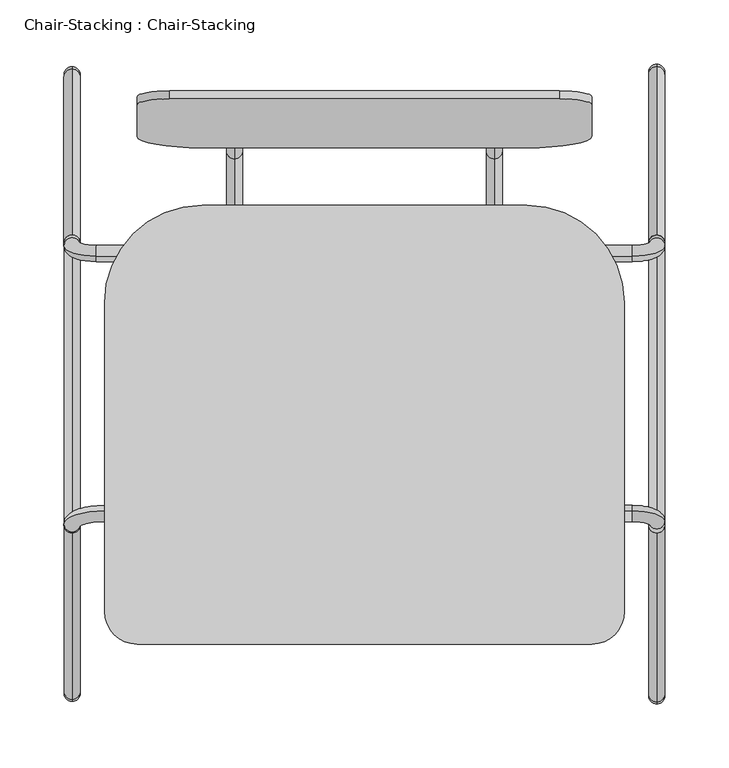
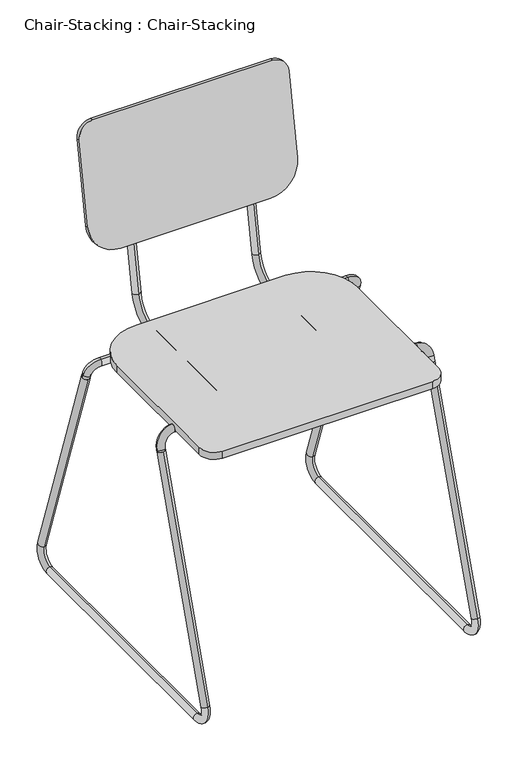
"""IFC4 building model written with IfcOpenShell, lengths in millimetres: furniture geometry, Chair-Stacking : Chair-Stacking."""

from ifc_helpers import new_model, si_unit, point, frame, frame_2d, origin, place, context, project, spatial, polyline, circle_curve, ellipse_curve, trimmed, segment, composite_curve, outline, extrude, source, transform, mapped, element, save
from ifc_brep_helpers import plane_surface, cylinder_surface, revolved_surface, advanced_brep


def chair_stacking_chair_stacking_89a83372(model_context):
    return source(origin(), model_context, "Body", "SolidModel", [
        advanced_brep(
        [(-280.6491803, -213.2656675, 431.8), (-280.6491803, -213.2656675, 444.5), (-280.6491803, 23.0277124, 444.5), (-280.6491803, 23.0277124, 431.8), (-280.6491803, 66.802417, 481.2313385), (-280.6491803, 79.3094755, 479.0260066), (-280.6491803, 119.2282049, 705.4163709), (-280.6491803, 106.7211464, 707.6217027)],
        [
            (0, 1, circle_curve(frame((-280.6491803, -213.2656675, 438.15), z_axis=(0.0, -1.0, 0.0), x_axis=(0.0, 0.0, 1.0)), 6.35)),
            (1, 0, circle_curve(frame((-280.6491803, -213.2656675, 438.15), z_axis=(0.0, -1.0, 0.0), x_axis=(0.0, 0.0, 1.0)), 6.35)),
            (1, 2),
            (2, 3, circle_curve(frame((-280.6491803, 23.0277124, 438.15), z_axis=(0.0, -1.0, 0.0), x_axis=(0.0, 0.0, 1.0)), 6.35)),
            (3, 0),
            (3, 2, circle_curve(frame((-280.6491803, 23.0277124, 438.15), z_axis=(0.0, -1.0, 0.0), x_axis=(0.0, 0.0, 1.0)), 6.35)),
            (4, 5, circle_curve(frame((-280.6491803, 73.0559463, 480.1286726), z_axis=(0.0, -0.17364817766693444, -0.9848077530122074), x_axis=(0.0, -0.9848077530122074, 0.17364817766693444)), 6.35)),
            (5, 3, circle_curve(frame((-280.6491803, 23.0277124, 488.95), z_axis=(-1.0, 0.0, 0.0), x_axis=(0.0, 0.0, -1.0)), 57.15)),
            (2, 4, circle_curve(frame((-280.6491803, 23.0277124, 488.95), z_axis=(1.0, 0.0, 0.0), x_axis=(0.0, 0.0, -1.0)), 44.45)),
            (5, 4, circle_curve(frame((-280.6491803, 73.0559463, 480.1286726), z_axis=(0.0, -0.17364817766693444, -0.9848077530122074), x_axis=(0.0, -0.9848077530122074, 0.17364817766693444)), 6.35)),
            (6, 7, circle_curve(frame((-280.6491803, 112.9746757, 706.5190368), z_axis=(0.0, 0.1736481776669348, 0.9848077530122074), x_axis=(0.0, -0.9848077530122074, 0.1736481776669348)), 6.35)),
            (7, 6, circle_curve(frame((-280.6491803, 112.9746757, 706.5190368), z_axis=(0.0, 0.1736481776669348, 0.9848077530122074), x_axis=(0.0, -0.9848077530122074, 0.1736481776669348)), 6.35)),
            (4, 7),
            (6, 5),
        ],
        [
            plane_surface(frame((-286.9991803, -213.2656675, 438.15), z_axis=(0.0, -1.0, 0.0), x_axis=(0.0, 0.0, -1.0))),
            cylinder_surface(frame((-280.6491803, -213.2656675, 438.15), z_axis=(0.0, -1.0, 0.0), x_axis=(0.0, 0.0, 1.0)), 6.35),
            revolved_surface(trimmed(ellipse_curve(frame((-280.6491803, 23.0277124, 438.15), z_axis=(0.0, 1.0, 0.0), x_axis=(0.0, 0.0, 1.0)), 6.35, 6.35), [point((-280.6491803, 23.0277124, 431.8))], [point((-280.6491803, 23.0277124, 444.5))], True, "CARTESIAN"), (-280.6491803, 23.0277124, 488.95), (-1.0, 0.0, 0.0)),
            revolved_surface(trimmed(ellipse_curve(frame((-280.6491803, 23.0277124, 438.15), z_axis=(0.0, 1.0, 0.0), x_axis=(0.0, 0.0, 1.0)), 6.35, 6.35), [point((-280.6491803, 23.0277124, 444.5))], [point((-280.6491803, 23.0277124, 431.8))], True, "CARTESIAN"), (-280.6491803, 23.0277124, 488.95), (-1.0, 0.0, 0.0)),
            plane_surface(frame((-280.6491803, 119.2282049, 705.4163709), z_axis=(0.0, 0.17364817766692842, 0.9848077530122085), x_axis=(1.0, 0.0, 0.0))),
            cylinder_surface(frame((-280.6491803, 73.0559463, 480.1286726), z_axis=(0.0, -0.1736481776669348, -0.9848077530122074), x_axis=(0.0, -0.9848077530122074, 0.1736481776669348)), 6.35),
        ],
        [
            (0, [[1, 2]]),
            (1, [[3, 4, 5, -2]]),
            (1, [[-5, 6, -3, -1]]),
            (2, [[7, 8, -4, 9]]),
            (3, [[10, -9, -6, -8]]),
            (4, [[11, 12]]),
            (5, [[13, -11, 14, -7]]),
            (5, [[-14, -12, -13, -10]]),
        ],
    ),
        advanced_brep(
        [(-77.4491803, -213.2656675, 431.8), (-77.4491803, -213.2656675, 444.5), (-77.4491803, 23.0277124, 444.5), (-77.4491803, 23.0277124, 431.8), (-77.4491803, 66.802417, 481.2313385), (-77.4491803, 79.3094755, 479.0260066), (-77.4491803, 118.9339087, 703.7473341), (-77.4491803, 106.4268502, 705.9526659)],
        [
            (0, 1, circle_curve(frame((-77.4491803, -213.2656675, 438.15), z_axis=(0.0, -1.0, 0.0), x_axis=(0.0, 0.0, 1.0)), 6.35)),
            (1, 0, circle_curve(frame((-77.4491803, -213.2656675, 438.15), z_axis=(0.0, -1.0, 0.0), x_axis=(0.0, 0.0, 1.0)), 6.35)),
            (1, 2),
            (2, 3, circle_curve(frame((-77.4491803, 23.0277124, 438.15), z_axis=(0.0, -1.0, 0.0), x_axis=(0.0, 0.0, 1.0)), 6.35)),
            (3, 0),
            (3, 2, circle_curve(frame((-77.4491803, 23.0277124, 438.15), z_axis=(0.0, -1.0, 0.0), x_axis=(0.0, 0.0, 1.0)), 6.35)),
            (4, 5, circle_curve(frame((-77.4491803, 73.0559463, 480.1286726), z_axis=(0.0, -0.1736481776669372, -0.9848077530122068), x_axis=(0.0, -0.9848077530122068, 0.1736481776669372)), 6.35)),
            (5, 3, circle_curve(frame((-77.4491803, 23.0277124, 488.95), z_axis=(-1.0, 0.0, 0.0), x_axis=(0.0, 0.0, -1.0)), 57.15)),
            (2, 4, circle_curve(frame((-77.4491803, 23.0277124, 488.95), z_axis=(1.0, 0.0, 0.0), x_axis=(0.0, 0.0, -1.0)), 44.45)),
            (5, 4, circle_curve(frame((-77.4491803, 73.0559463, 480.1286726), z_axis=(0.0, -0.1736481776669385, -0.9848077530122066), x_axis=(0.0, -0.9848077530122066, 0.1736481776669385)), 6.35)),
            (6, 7, circle_curve(frame((-77.4491803, 112.6803794, 704.85), z_axis=(0.0, 0.17364817766693896, 0.9848077530122066), x_axis=(0.0, -0.9848077530122066, 0.17364817766693896)), 6.35)),
            (7, 6, circle_curve(frame((-77.4491803, 112.6803794, 704.85), z_axis=(0.0, 0.17364817766693896, 0.9848077530122066), x_axis=(0.0, -0.9848077530122066, 0.17364817766693896)), 6.35)),
            (4, 7),
            (6, 5),
        ],
        [
            plane_surface(frame((-83.7991803, -213.2656675, 438.15), z_axis=(0.0, -1.0, 0.0), x_axis=(0.0, 0.0, -1.0))),
            cylinder_surface(frame((-77.4491803, -213.2656675, 438.15), z_axis=(0.0, -1.0, 0.0), x_axis=(0.0, 0.0, 1.0)), 6.35),
            revolved_surface(trimmed(ellipse_curve(frame((-77.4491803, 23.0277124, 438.15), z_axis=(0.0, 1.0, 0.0), x_axis=(0.0, 0.0, 1.0)), 6.35, 6.35), [point((-77.4491803, 23.0277124, 431.8))], [point((-77.4491803, 23.0277124, 444.5))], True, "CARTESIAN"), (-77.4491803, 23.0277124, 488.95), (-1.0, 0.0, 0.0)),
            revolved_surface(trimmed(ellipse_curve(frame((-77.4491803, 23.0277124, 438.15), z_axis=(0.0, 1.0, 0.0), x_axis=(0.0, 0.0, 1.0)), 6.35, 6.35), [point((-77.4491803, 23.0277124, 444.5))], [point((-77.4491803, 23.0277124, 431.8))], True, "CARTESIAN"), (-77.4491803, 23.0277124, 488.95), (-1.0, 0.0, 0.0)),
            plane_surface(frame((-77.4491803, 118.9339087, 703.7473341), z_axis=(0.0, 0.17364817766692892, 0.9848077530122084), x_axis=(1.0, 0.0, 0.0))),
            cylinder_surface(frame((-77.4491803, 73.0559463, 480.1286726), z_axis=(0.0, -0.17364817766693896, -0.9848077530122066), x_axis=(0.0, -0.9848077530122066, 0.17364817766693896)), 6.35),
        ],
        [
            (0, [[1, 2]]),
            (1, [[3, 4, 5, -2]]),
            (1, [[-5, 6, -3, -1]]),
            (2, [[7, 8, -4, 9]]),
            (3, [[10, -9, -6, -8]]),
            (4, [[11, 12]]),
            (5, [[13, -11, 14, -7]]),
            (5, [[-14, -12, -13, -10]]),
        ],
    ),
        extrude(outline(composite_curve([segment(polyline([(-1.2491803, -312.1314636), (-356.8491803, -312.1314636)]), True, "CONTINUOUS"), segment(trimmed(circle_curve(frame_2d((-356.8491803, -286.7314636)), 25.4), [point((-356.8491803, -312.1314636))], [point((-382.2491803, -286.7314636))], False, "CARTESIAN"), True, "CONTINUOUS"), segment(polyline([(-382.2491803, -286.7314636), (-382.2491803, -45.4314636)]), True, "CONTINUOUS"), segment(trimmed(circle_curve(frame_2d((-306.0491803, -45.4314636)), 76.2), [point((-382.2491803, -45.4314636))], [point((-306.0491803, 30.7685364))], False, "CARTESIAN"), True, "CONTINUOUS"), segment(polyline([(-306.0491803, 30.7685364), (-52.0491803, 30.7685364)]), True, "CONTINUOUS"), segment(trimmed(circle_curve(frame_2d((-52.0491803, -45.4314636)), 76.2), [point((-52.0491803, 30.7685364))], [point((24.1508197, -45.4314636))], False, "CARTESIAN"), True, "CONTINUOUS"), segment(polyline([(24.1508197, -45.4314636), (24.1508197, -286.7314636)]), True, "CONTINUOUS"), segment(trimmed(circle_curve(frame_2d((-1.2491803, -286.7314636)), 25.4), [point((24.1508197, -286.7314636))], [point((-1.2491803, -312.1314636))], False, "CARTESIAN"), True, "CONTINUOUS")], self_intersect=False)), frame((0.0, 0.0, 444.5), z_axis=(0.0, 0.0, 1.0), x_axis=(1.0, 0.0, 0.0)), (0.0, 0.0, 1.0), 12.7),
        extrude(outline(composite_curve([segment(trimmed(circle_curve(frame_2d((-304.8, 25.4)), 25.4), [point((-304.8, 0.0))], [point((-330.2, 25.4))], False, "CARTESIAN"), True, "CONTINUOUS"), segment(polyline([(-330.2, 25.4), (-330.2, 168.3013626)]), True, "CONTINUOUS"), segment(trimmed(circle_curve(frame_2d((-279.4, 168.3013626)), 50.8), [point((-330.2, 168.3013626))], [point((-279.4, 219.1013626))], False, "CARTESIAN"), True, "CONTINUOUS"), segment(polyline([(-279.4, 219.1013626), (-25.4, 219.1013626)]), True, "CONTINUOUS"), segment(trimmed(circle_curve(frame_2d((-25.4, 168.3013626)), 50.8), [point((-25.4, 219.1013626))], [point((25.4, 168.3013626))], False, "CARTESIAN"), True, "CONTINUOUS"), segment(polyline([(25.4, 168.3013626), (25.4, 25.4)]), True, "CONTINUOUS"), segment(trimmed(circle_curve(frame_2d((0.0, 25.4)), 25.4), [point((25.4, 25.4))], [point((0.0, 0.0))], False, "CARTESIAN"), True, "CONTINUOUS"), segment(polyline([(0.0, 0.0), (-304.8, 0.0)]), True, "CONTINUOUS")], self_intersect=False)), frame((-331.4491803, 119.9531376, 782.6640535), z_axis=(0.0, -0.9848077530122084, 0.17364817766692858), x_axis=(-1.0, 0.0, 0.0)), (0.0, 0.0, 1.0), 6.35),
        advanced_brep(
        [(55.9008197, -219.2327758, 419.1211728), (43.2008197, -219.2327758, 419.1211728), (43.2008197, -216.3017292, 427.6700586), (55.9008197, -216.3017292, 427.6700586), (30.5008197, -212.1828103, 439.6835721), (30.5008197, -208.0638914, 451.6970857), (-382.2491803, -212.1828103, 439.6835721), (-382.2491803, -208.0638914, 451.6970857), (-401.2991803, -218.3611887, 421.6633019), (-413.9991803, -218.3611887, 421.6633019), (-413.9991803, -219.2424531, 419.0929473), (-401.2991803, -219.2424531, 419.0929473)],
        [
            (0, 1, circle_curve(frame((49.5508197, -219.2327758, 419.1211728), z_axis=(0.0, -0.32432432432432967, -0.9459459459459442), x_axis=(-1.0, 0.0, 0.0)), 6.35)),
            (1, 0, circle_curve(frame((49.5508197, -219.2327758, 419.1211728), z_axis=(0.0, -0.32432432432432967, -0.9459459459459442), x_axis=(-1.0, 0.0, 0.0)), 6.35)),
            (1, 2),
            (2, 3, circle_curve(frame((49.5508197, -216.3017292, 427.6700586), z_axis=(0.0, -0.32432432432432967, -0.9459459459459442), x_axis=(-1.0, 0.0, 0.0)), 6.35)),
            (3, 0),
            (3, 2, circle_curve(frame((49.5508197, -216.3017292, 427.6700586), z_axis=(0.0, -0.32432432432432967, -0.9459459459459442), x_axis=(-1.0, 0.0, 0.0)), 6.35)),
            (4, 5, circle_curve(frame((30.5008197, -210.1233509, 445.6903289), z_axis=(1.0, 0.0, 0.0), x_axis=(0.0, -0.32432432432432745, -0.9459459459459449)), 6.35)),
            (5, 3, circle_curve(frame((30.5008197, -216.3017292, 427.6700586), z_axis=(0.0, 0.9459459459459447, -0.3243243243243281), x_axis=(1.0, 0.0, 0.0)), 25.4)),
            (2, 4, circle_curve(frame((30.5008197, -216.3017292, 427.6700586), z_axis=(0.0, -0.9459459459459447, 0.3243243243243281), x_axis=(1.0, 0.0, 0.0)), 12.7)),
            (5, 4, circle_curve(frame((30.5008197, -210.1233509, 445.6903289), z_axis=(1.0, 0.0, 0.0), x_axis=(0.0, -0.32432432432432745, -0.9459459459459449)), 6.35)),
            (4, 6),
            (6, 7, circle_curve(frame((-382.2491803, -210.1233509, 445.6903289), z_axis=(1.0, 0.0, 0.0), x_axis=(0.0, -0.32432432432432745, -0.9459459459459449)), 6.35)),
            (7, 5),
            (7, 6, circle_curve(frame((-382.2491803, -210.1233509, 445.6903289), z_axis=(1.0, 0.0, 0.0), x_axis=(0.0, -0.32432432432432745, -0.9459459459459449)), 6.35)),
            (8, 9, circle_curve(frame((-407.6491803, -218.3611887, 421.6633019), z_axis=(0.0, 0.324324324324328, 0.9459459459459447), x_axis=(1.0000000000000002, 0.0, 0.0)), 6.35)),
            (9, 7, circle_curve(frame((-382.2491803, -218.3611887, 421.6633019), z_axis=(0.0, 0.9459459459459447, -0.3243243243243281), x_axis=(0.0, 0.3243243243243281, 0.9459459459459447)), 31.75)),
            (6, 8, circle_curve(frame((-382.2491803, -218.3611887, 421.6633019), z_axis=(0.0, -0.9459459459459447, 0.3243243243243281), x_axis=(0.0, 0.3243243243243281, 0.9459459459459447)), 19.05)),
            (9, 8, circle_curve(frame((-407.6491803, -218.3611887, 421.6633019), z_axis=(0.0, 0.324324324324328, 0.9459459459459447), x_axis=(1.0000000000000002, 0.0, 0.0)), 6.35)),
            (10, 11, circle_curve(frame((-407.6491803, -219.2424531, 419.0929473), z_axis=(0.0, -0.32432432432432784, -0.9459459459459449), x_axis=(1.0, 0.0, 0.0)), 6.35)),
            (11, 10, circle_curve(frame((-407.6491803, -219.2424531, 419.0929473), z_axis=(0.0, -0.32432432432432784, -0.9459459459459449), x_axis=(1.0, 0.0, 0.0)), 6.35)),
            (8, 11),
            (10, 9),
        ],
        [
            plane_surface(frame((49.5508197, -213.226019, 417.0617133), z_axis=(0.0, -0.32432432432433117, -0.9459459459459437), x_axis=(1.0, 0.0, 0.0))),
            cylinder_surface(frame((49.5508197, -219.2327758, 419.1211728), z_axis=(0.0, -0.32432432432432967, -0.9459459459459442), x_axis=(-1.0, 0.0, 0.0)), 6.35),
            revolved_surface(trimmed(ellipse_curve(frame((49.5508197, -216.3017292, 427.6700586), z_axis=(0.0, 0.32432432432432823, 0.9459459459459447), x_axis=(-1.0, 0.0, 0.0)), 6.35, 6.35), [point((55.9008197, -216.3017292, 427.6700586))], [point((43.2008197, -216.3017292, 427.6700586))], True, "CARTESIAN"), (30.5008197, -216.3017292, 427.6700586), (0.0, 0.9459459459459447, -0.3243243243243281)),
            revolved_surface(trimmed(ellipse_curve(frame((49.5508197, -216.3017292, 427.6700586), z_axis=(0.0, 0.32432432432432823, 0.9459459459459447), x_axis=(-1.0, 0.0, 0.0)), 6.35, 6.35), [point((43.2008197, -216.3017292, 427.6700586))], [point((55.9008197, -216.3017292, 427.6700586))], True, "CARTESIAN"), (30.5008197, -216.3017292, 427.6700586), (0.0, 0.9459459459459447, -0.3243243243243281)),
            cylinder_surface(frame((30.5008197, -210.1233509, 445.6903289), z_axis=(1.0, 0.0, 0.0), x_axis=(0.0, -0.32432432432432745, -0.9459459459459449)), 6.35),
            revolved_surface(trimmed(ellipse_curve(frame((-382.2491803, -210.1233509, 445.6903289), z_axis=(-1.0000000000000002, 0.0, 0.0), x_axis=(0.0, -0.3243243243243276, -0.9459459459459449)), 6.35, 6.35), [point((-382.2491803, -208.0638914, 451.6970857))], [point((-382.2491803, -212.1828103, 439.6835721))], True, "CARTESIAN"), (-382.2491803, -218.3611887, 421.6633019), (0.0, 0.9459459459459447, -0.3243243243243281)),
            revolved_surface(trimmed(ellipse_curve(frame((-382.2491803, -210.1233509, 445.6903289), z_axis=(-1.0000000000000002, 0.0, 0.0), x_axis=(0.0, -0.3243243243243276, -0.9459459459459449)), 6.35, 6.35), [point((-382.2491803, -212.1828103, 439.6835721))], [point((-382.2491803, -208.0638914, 451.6970857))], True, "CARTESIAN"), (-382.2491803, -218.3611887, 421.6633019), (0.0, 0.9459459459459447, -0.3243243243243281)),
            plane_surface(frame((-407.6491803, -225.2492099, 421.1524068), z_axis=(0.0, -0.3243243243243264, -0.9459459459459453), x_axis=(1.0, 0.0, 0.0))),
            cylinder_surface(frame((-407.6491803, -218.3611887, 421.6633019), z_axis=(0.0, 0.3243243243243278, 0.9459459459459447), x_axis=(1.0, 0.0, 0.0)), 6.35),
        ],
        [
            (0, [[1, 2]]),
            (1, [[3, 4, 5, -2]]),
            (1, [[-5, 6, -3, -1]]),
            (2, [[7, 8, -4, 9]]),
            (3, [[10, -9, -6, -8]]),
            (4, [[11, 12, 13, -7]]),
            (4, [[-13, 14, -11, -10]]),
            (5, [[15, 16, -12, 17]]),
            (6, [[18, -17, -14, -16]]),
            (7, [[19, 20]]),
            (8, [[21, -19, 22, -15]]),
            (8, [[-22, -20, -21, -18]]),
        ],
    ),
        advanced_brep(
        [(55.9008197, 1.3812406, 419.0879461), (43.2008197, 1.3812406, 419.0879461), (43.2008197, -0.7944914, 425.4338312), (55.9008197, -0.7944914, 425.4338312), (30.5008197, -4.9134104, 437.4473447), (30.5008197, -9.0323293, 449.4608582), (-388.5991803, -4.9134104, 437.4473447), (-388.5991803, -9.0323293, 449.4608582), (-401.2991803, -0.7944914, 425.4338312), (-413.9991803, -0.7944914, 425.4338312), (-413.9991803, 1.3997864, 419.0338542), (-401.2991803, 1.3997864, 419.0338542)],
        [
            (0, 1, circle_curve(frame((49.5508197, 1.3812406, 419.0879461), z_axis=(0.0, 0.32432432432432495, -0.9459459459459457), x_axis=(-1.0, 0.0, 0.0)), 6.35)),
            (1, 0, circle_curve(frame((49.5508197, 1.3812406, 419.0879461), z_axis=(0.0, 0.32432432432432495, -0.9459459459459457), x_axis=(-1.0, 0.0, 0.0)), 6.35)),
            (1, 2),
            (2, 3, circle_curve(frame((49.5508197, -0.7944914, 425.4338312), z_axis=(0.0, 0.32432432432432495, -0.9459459459459457), x_axis=(-1.0, 0.0, 0.0)), 6.35)),
            (3, 0),
            (3, 2, circle_curve(frame((49.5508197, -0.7944914, 425.4338312), z_axis=(0.0, 0.32432432432432495, -0.9459459459459457), x_axis=(-1.0, 0.0, 0.0)), 6.35)),
            (4, 5, circle_curve(frame((30.5008197, -6.9728698, 443.4541014), z_axis=(1.0, 0.0, 0.0), x_axis=(0.0, 0.3243243243243236, -0.9459459459459462)), 6.35)),
            (5, 3, circle_curve(frame((30.5008197, -0.7944914, 425.4338312), z_axis=(0.0, 0.9459459459459458, 0.3243243243243246), x_axis=(1.0, 0.0, 0.0)), 25.4)),
            (2, 4, circle_curve(frame((30.5008197, -0.7944914, 425.4338312), z_axis=(0.0, -0.9459459459459458, -0.3243243243243246), x_axis=(1.0, 0.0, 0.0)), 12.7)),
            (5, 4, circle_curve(frame((30.5008197, -6.9728698, 443.4541014), z_axis=(1.0, 0.0, 0.0), x_axis=(0.0, 0.3243243243243236, -0.9459459459459462)), 6.35)),
            (4, 6),
            (6, 7, circle_curve(frame((-388.5991803, -6.9728698, 443.4541014), z_axis=(1.0, 0.0, 0.0), x_axis=(0.0, 0.3243243243243236, -0.9459459459459462)), 6.35)),
            (7, 5),
            (7, 6, circle_curve(frame((-388.5991803, -6.9728698, 443.4541014), z_axis=(1.0, 0.0, 0.0), x_axis=(0.0, 0.3243243243243236, -0.9459459459459462)), 6.35)),
            (8, 9, circle_curve(frame((-407.6491803, -0.7944914, 425.4338312), z_axis=(0.0, -0.3243243243243247, 0.9459459459459458), x_axis=(1.0, 0.0, 0.0)), 6.35)),
            (9, 7, circle_curve(frame((-388.5991803, -0.7944914, 425.4338312), z_axis=(0.0, 0.9459459459459458, 0.3243243243243246), x_axis=(0.0, -0.3243243243243246, 0.9459459459459458)), 25.4)),
            (6, 8, circle_curve(frame((-388.5991803, -0.7944914, 425.4338312), z_axis=(0.0, -0.9459459459459458, -0.3243243243243246), x_axis=(0.0, -0.3243243243243246, 0.9459459459459458)), 12.7)),
            (9, 8, circle_curve(frame((-407.6491803, -0.7944914, 425.4338312), z_axis=(0.0, -0.3243243243243247, 0.9459459459459458), x_axis=(1.0, 0.0, 0.0)), 6.35)),
            (10, 11, circle_curve(frame((-407.6491803, 1.3997864, 419.0338542), z_axis=(0.0, 0.3243243243243242, -0.945945945945946), x_axis=(1.0, 0.0, 0.0)), 6.35)),
            (11, 10, circle_curve(frame((-407.6491803, 1.3997864, 419.0338542), z_axis=(0.0, 0.3243243243243242, -0.945945945945946), x_axis=(1.0, 0.0, 0.0)), 6.35)),
            (8, 11),
            (10, 9),
        ],
        [
            plane_surface(frame((49.5508197, 7.3879973, 421.1474055), z_axis=(0.0, 0.32432432432432273, -0.9459459459459466), x_axis=(1.0, 0.0, 0.0))),
            cylinder_surface(frame((49.5508197, 1.3812406, 419.0879461), z_axis=(0.0, 0.32432432432432495, -0.9459459459459457), x_axis=(-1.0, 0.0, 0.0)), 6.35),
            revolved_surface(trimmed(ellipse_curve(frame((49.5508197, -0.7944914, 425.4338312), z_axis=(0.0, -0.32432432432432456, 0.9459459459459458), x_axis=(-1.0, 0.0, 0.0)), 6.35, 6.35), [point((55.9008197, -0.7944914, 425.4338312))], [point((43.2008197, -0.7944914, 425.4338312))], True, "CARTESIAN"), (30.5008197, -0.7944914, 425.4338312), (0.0, 0.9459459459459458, 0.3243243243243246)),
            revolved_surface(trimmed(ellipse_curve(frame((49.5508197, -0.7944914, 425.4338312), z_axis=(0.0, -0.32432432432432456, 0.9459459459459458), x_axis=(-1.0, 0.0, 0.0)), 6.35, 6.35), [point((43.2008197, -0.7944914, 425.4338312))], [point((55.9008197, -0.7944914, 425.4338312))], True, "CARTESIAN"), (30.5008197, -0.7944914, 425.4338312), (0.0, 0.9459459459459458, 0.3243243243243246)),
            cylinder_surface(frame((30.5008197, -6.9728698, 443.4541014), z_axis=(1.0, 0.0, 0.0), x_axis=(0.0, 0.3243243243243236, -0.9459459459459462)), 6.35),
            revolved_surface(trimmed(ellipse_curve(frame((-388.5991803, -6.9728698, 443.4541014), z_axis=(-1.0, 0.0, 0.0), x_axis=(0.0, 0.3243243243243236, -0.9459459459459462)), 6.35, 6.35), [point((-388.5991803, -9.0323293, 449.4608582))], [point((-388.5991803, -4.9134104, 437.4473447))], True, "CARTESIAN"), (-388.5991803, -0.7944914, 425.4338312), (0.0, 0.9459459459459458, 0.3243243243243246)),
            revolved_surface(trimmed(ellipse_curve(frame((-388.5991803, -6.9728698, 443.4541014), z_axis=(-1.0, 0.0, 0.0), x_axis=(0.0, 0.3243243243243236, -0.9459459459459462)), 6.35, 6.35), [point((-388.5991803, -4.9134104, 437.4473447))], [point((-388.5991803, -9.0323293, 449.4608582))], True, "CARTESIAN"), (-388.5991803, -0.7944914, 425.4338312), (0.0, 0.9459459459459458, 0.3243243243243246)),
            plane_surface(frame((-407.6491803, -4.6069704, 416.9743947), z_axis=(0.0, 0.3243243243243226, -0.9459459459459466), x_axis=(1.0, 0.0, 0.0))),
            cylinder_surface(frame((-407.6491803, -0.7944914, 425.4338312), z_axis=(0.0, -0.3243243243243242, 0.945945945945946), x_axis=(1.0, 0.0, 0.0)), 6.35),
        ],
        [
            (0, [[1, 2]]),
            (1, [[3, 4, 5, -2]]),
            (1, [[-5, 6, -3, -1]]),
            (2, [[7, 8, -4, 9]]),
            (3, [[10, -9, -6, -8]]),
            (4, [[11, 12, 13, -7]]),
            (4, [[-13, 14, -11, -10]]),
            (5, [[15, 16, -12, 17]]),
            (6, [[18, -17, -14, -16]]),
            (7, [[19, 20]]),
            (8, [[21, -19, 22, -15]]),
            (8, [[-22, -20, -21, -18]]),
        ],
    ),
        advanced_brep(
        [(-407.6491803, -225.2492099, 421.1524068), (-407.6491803, -213.2356963, 417.0334879), (-407.6491803, -343.214591, 37.9283784), (-407.6491803, -355.2281045, 42.0472973), (-407.6491803, -325.1943208, 12.7), (-407.6491803, -325.1943208, 0.0), (-407.6491803, 107.3313935, 12.7), (-407.6491803, 107.3313935, 0.0), (-407.6491803, 125.3516638, 37.9283784), (-407.6491803, 137.3651773, 42.0472973), (-407.6491803, 7.4065431, 421.0933136), (-407.6491803, -4.6069704, 416.9743947)],
        [
            (0, 1, circle_curve(frame((-407.6491803, -219.2424531, 419.0929473), z_axis=(0.0, 0.3243243243243311, 0.9459459459459437), x_axis=(0.0, 0.9459459459459437, -0.3243243243243311)), 6.35)),
            (1, 0, circle_curve(frame((-407.6491803, -219.2424531, 419.0929473), z_axis=(0.0, 0.3243243243243311, 0.9459459459459437), x_axis=(0.0, 0.9459459459459437, -0.3243243243243311)), 6.35)),
            (1, 2),
            (2, 3, circle_curve(frame((-407.6491803, -349.2213478, 39.9878378), z_axis=(0.0, 0.3243243243243311, 0.9459459459459437), x_axis=(0.0, 0.9459459459459437, -0.3243243243243311)), 6.35)),
            (3, 0),
            (3, 2, circle_curve(frame((-407.6491803, -349.2213478, 39.9878378), z_axis=(0.0, 0.3243243243243311, 0.9459459459459437), x_axis=(0.0, 0.9459459459459437, -0.3243243243243311)), 6.35)),
            (4, 5, circle_curve(frame((-407.6491803, -325.1943208, 6.35), z_axis=(0.0, -0.9999999999999999, 0.0), x_axis=(0.0, 0.0, 0.9999999999999999)), 6.35)),
            (5, 3, circle_curve(frame((-407.6491803, -325.1943208, 31.75), z_axis=(-1.0, 0.0, 0.0), x_axis=(0.0, -0.9459459459459434, 0.3243243243243317)), 31.75)),
            (2, 4, circle_curve(frame((-407.6491803, -325.1943208, 31.75), z_axis=(1.0, 0.0, 0.0), x_axis=(0.0, -0.9459459459459434, 0.3243243243243317)), 19.05)),
            (5, 4, circle_curve(frame((-407.6491803, -325.1943208, 6.35), z_axis=(0.0, -1.0, 0.0), x_axis=(0.0, 0.0, 1.0)), 6.35)),
            (4, 6),
            (6, 7, circle_curve(frame((-407.6491803, 107.3313935, 6.35), z_axis=(0.0, -1.0, 0.0), x_axis=(0.0, 0.0, 1.0)), 6.35)),
            (7, 5),
            (7, 6, circle_curve(frame((-407.6491803, 107.3313935, 6.35), z_axis=(0.0, -1.0, 0.0), x_axis=(0.0, 0.0, 1.0)), 6.35)),
            (8, 9, circle_curve(frame((-407.6491803, 131.3584206, 39.9878378), z_axis=(0.0, 0.3243243243243206, -0.9459459459459473), x_axis=(0.0, -0.9459459459459473, -0.3243243243243206)), 6.35)),
            (9, 7, circle_curve(frame((-407.6491803, 107.3313935, 31.75), z_axis=(-1.0, 0.0, 0.0), x_axis=(0.0, 0.0, -1.0)), 31.75)),
            (6, 8, circle_curve(frame((-407.6491803, 107.3313935, 31.75), z_axis=(1.0, 0.0, 0.0), x_axis=(0.0, 0.0, -1.0)), 19.05)),
            (9, 8, circle_curve(frame((-407.6491803, 131.3584206, 39.9878378), z_axis=(0.0, 0.3243243243243189, -0.9459459459459478), x_axis=(0.0, -0.9459459459459478, -0.3243243243243189)), 6.35)),
            (10, 11, circle_curve(frame((-407.6491803, 1.3997864, 419.0338542), z_axis=(0.0, -0.3243243243243217, 0.9459459459459468), x_axis=(0.0, -0.9459459459459468, -0.3243243243243217)), 6.35)),
            (11, 10, circle_curve(frame((-407.6491803, 1.3997864, 419.0338542), z_axis=(0.0, -0.3243243243243217, 0.9459459459459468), x_axis=(0.0, -0.9459459459459468, -0.3243243243243217)), 6.35)),
            (8, 11),
            (10, 9),
        ],
        [
            plane_surface(frame((-407.6491803, -225.2492099, 421.1524068), z_axis=(0.0, 0.32432432432432773, 0.9459459459459448), x_axis=(1.0, 0.0, 0.0))),
            cylinder_surface(frame((-407.6491803, -219.2424531, 419.0929473), z_axis=(0.0, 0.3243243243243311, 0.9459459459459437), x_axis=(0.0, 0.9459459459459437, -0.3243243243243311)), 6.35),
            revolved_surface(trimmed(ellipse_curve(frame((-407.6491803, -349.2213478, 39.9878378), z_axis=(0.0, -0.3243243243243347, -0.9459459459459424), x_axis=(0.0, 0.9459459459459424, -0.3243243243243347)), 6.35, 6.35), [point((-407.6491803, -355.2281045, 42.0472973))], [point((-407.6491803, -343.214591, 37.9283784))], True, "CARTESIAN"), (-407.6491803, -325.1943208, 31.75), (-1.0, 0.0, 0.0)),
            revolved_surface(trimmed(ellipse_curve(frame((-407.6491803, -349.2213478, 39.9878378), z_axis=(0.0, -0.3243243243243347, -0.9459459459459424), x_axis=(0.0, 0.9459459459459424, -0.3243243243243347)), 6.35, 6.35), [point((-407.6491803, -343.214591, 37.9283784))], [point((-407.6491803, -355.2281045, 42.0472973))], True, "CARTESIAN"), (-407.6491803, -325.1943208, 31.75), (-1.0, 0.0, 0.0)),
            cylinder_surface(frame((-407.6491803, -325.1943208, 6.35), z_axis=(0.0, -1.0, 0.0), x_axis=(0.0, 0.0, 1.0)), 6.35),
            revolved_surface(trimmed(ellipse_curve(frame((-407.6491803, 107.3313935, 6.35), z_axis=(0.0, 1.0, 0.0), x_axis=(0.0, 0.0, 1.0)), 6.35, 6.35), [point((-407.6491803, 107.3313935, 0.0))], [point((-407.6491803, 107.3313935, 12.7))], True, "CARTESIAN"), (-407.6491803, 107.3313935, 31.75), (-1.0, 0.0, 0.0)),
            revolved_surface(trimmed(ellipse_curve(frame((-407.6491803, 107.3313935, 6.35), z_axis=(0.0, 1.0, 0.0), x_axis=(0.0, 0.0, 1.0)), 6.35, 6.35), [point((-407.6491803, 107.3313935, 12.7))], [point((-407.6491803, 107.3313935, 0.0))], True, "CARTESIAN"), (-407.6491803, 107.3313935, 31.75), (-1.0, 0.0, 0.0)),
            plane_surface(frame((-407.6491803, 7.4065431, 421.0933136), z_axis=(0.0, -0.324324324324323, 0.9459459459459465), x_axis=(1.0, 0.0, 0.0))),
            cylinder_surface(frame((-407.6491803, 131.3584206, 39.9878378), z_axis=(0.0, 0.3243243243243217, -0.9459459459459468), x_axis=(0.0, -0.9459459459459468, -0.3243243243243217)), 6.35),
        ],
        [
            (0, [[1, 2]]),
            (1, [[3, 4, 5, -2]]),
            (1, [[-5, 6, -3, -1]]),
            (2, [[7, 8, -4, 9]]),
            (3, [[10, -9, -6, -8]]),
            (4, [[11, 12, 13, -7]]),
            (4, [[-13, 14, -11, -10]]),
            (5, [[15, 16, -12, 17]]),
            (6, [[18, -17, -14, -16]]),
            (7, [[19, 20]]),
            (8, [[21, -19, 22, -15]]),
            (8, [[-22, -20, -21, -18]]),
        ],
    ),
        advanced_brep(
        [(49.5508197, -225.2597598, 421.1875673), (49.5508197, -213.2656675, 417.0124327), (49.5508197, -345.1951918, 38.0127019), (49.5508197, -357.1892841, 42.1878365), (49.5508197, -327.2040533, 12.7), (49.5508197, -327.2040533, 0.0), (49.5508197, 109.3411268, 12.7), (49.5508197, 109.3411268, 0.0), (49.5508197, 127.3337908, 38.0083179), (49.5508197, 139.3289001, 42.1805298), (49.5508197, 7.5008737, 421.186106), (49.5508197, -4.4942357, 417.013894)],
        [
            (0, 1, circle_curve(frame((49.5508197, -219.2627136, 419.1), z_axis=(0.0, 0.3287507573582007, 0.9444167192168982), x_axis=(0.0, 0.9444167192168982, -0.3287507573582007)), 6.35)),
            (1, 0, circle_curve(frame((49.5508197, -219.2627136, 419.1), z_axis=(0.0, 0.3287507573582007, 0.9444167192168982), x_axis=(0.0, 0.9444167192168982, -0.3287507573582007)), 6.35)),
            (1, 2),
            (2, 3, circle_curve(frame((49.5508197, -351.1922379, 40.1002692), z_axis=(0.0, 0.3287507573582007, 0.9444167192168982), x_axis=(0.0, 0.9444167192168982, -0.3287507573582007)), 6.35)),
            (3, 0),
            (3, 2, circle_curve(frame((49.5508197, -351.1922379, 40.1002692), z_axis=(0.0, 0.3287507573582007, 0.9444167192168982), x_axis=(0.0, 0.9444167192168982, -0.3287507573582007)), 6.35)),
            (4, 5, circle_curve(frame((49.5508197, -327.2040533, 6.35), z_axis=(0.0, -0.9999999999999999, 0.0), x_axis=(0.0, 0.0, 0.9999999999999999)), 6.35)),
            (5, 3, circle_curve(frame((49.5508197, -327.2040533, 31.75), z_axis=(-1.0, 0.0, 0.0), x_axis=(0.0, -0.944416719216897, 0.3287507573582041)), 31.75)),
            (2, 4, circle_curve(frame((49.5508197, -327.2040533, 31.75), z_axis=(1.0, 0.0, 0.0), x_axis=(0.0, -0.944416719216897, 0.3287507573582041)), 19.05)),
            (5, 4, circle_curve(frame((49.5508197, -327.2040533, 6.35), z_axis=(0.0, -1.0, 0.0), x_axis=(0.0, 0.0, 1.0)), 6.35)),
            (4, 6),
            (6, 7, circle_curve(frame((49.5508197, 109.3411268, 6.35), z_axis=(0.0, -1.0, 0.0), x_axis=(0.0, 0.0, 1.0)), 6.35)),
            (7, 5),
            (7, 6, circle_curve(frame((49.5508197, 109.3411268, 6.35), z_axis=(0.0, -1.0, 0.0), x_axis=(0.0, 0.0, 1.0)), 6.35)),
            (8, 9, circle_curve(frame((49.5508197, 133.3313455, 40.0944239), z_axis=(0.0, 0.3285206249412754, -0.9444967967061582), x_axis=(0.0, -0.9444967967061582, -0.3285206249412754)), 6.35)),
            (9, 7, circle_curve(frame((49.5508197, 109.3411268, 31.75), z_axis=(-1.0, 0.0, 0.0), x_axis=(0.0, 0.0, -1.0)), 31.75)),
            (6, 8, circle_curve(frame((49.5508197, 109.3411268, 31.75), z_axis=(1.0, 0.0, 0.0), x_axis=(0.0, 0.0, -1.0)), 19.05)),
            (9, 8, circle_curve(frame((49.5508197, 133.3313455, 40.0944239), z_axis=(0.0, 0.3285206249412718, -0.9444967967061594), x_axis=(0.0, -0.9444967967061594, -0.3285206249412718)), 6.35)),
            (10, 11, circle_curve(frame((49.5508197, 1.503319, 419.1), z_axis=(0.0, -0.3285206249412728, 0.9444967967061592), x_axis=(0.0, -0.9444967967061592, -0.3285206249412728)), 6.35)),
            (11, 10, circle_curve(frame((49.5508197, 1.503319, 419.1), z_axis=(0.0, -0.3285206249412728, 0.9444967967061592), x_axis=(0.0, -0.9444967967061592, -0.3285206249412728)), 6.35)),
            (8, 11),
            (10, 9),
        ],
        [
            plane_surface(frame((49.5508197, -225.2597598, 421.1875673), z_axis=(0.0, 0.3287507573582023, 0.9444167192168977), x_axis=(1.0, 0.0, 0.0))),
            cylinder_surface(frame((49.5508197, -219.2627136, 419.1), z_axis=(0.0, 0.3287507573582007, 0.9444167192168982), x_axis=(0.0, 0.9444167192168982, -0.3287507573582007)), 6.35),
            revolved_surface(trimmed(ellipse_curve(frame((49.5508197, -351.1922379, 40.1002692), z_axis=(0.0, -0.32875075735820414, -0.944416719216897), x_axis=(0.0, 0.944416719216897, -0.32875075735820414)), 6.35, 6.35), [point((49.5508197, -357.1892841, 42.1878365))], [point((49.5508197, -345.1951918, 38.0127019))], True, "CARTESIAN"), (49.5508197, -327.2040533, 31.75), (-1.0, 0.0, 0.0)),
            revolved_surface(trimmed(ellipse_curve(frame((49.5508197, -351.1922379, 40.1002692), z_axis=(0.0, -0.32875075735820414, -0.944416719216897), x_axis=(0.0, 0.944416719216897, -0.32875075735820414)), 6.35, 6.35), [point((49.5508197, -345.1951918, 38.0127019))], [point((49.5508197, -357.1892841, 42.1878365))], True, "CARTESIAN"), (49.5508197, -327.2040533, 31.75), (-1.0, 0.0, 0.0)),
            cylinder_surface(frame((49.5508197, -327.2040533, 6.35), z_axis=(0.0, -1.0, 0.0), x_axis=(0.0, 0.0, 1.0)), 6.35),
            revolved_surface(trimmed(ellipse_curve(frame((49.5508197, 109.3411268, 6.35), z_axis=(0.0, 1.0, 0.0), x_axis=(0.0, 0.0, 1.0)), 6.35, 6.35), [point((49.5508197, 109.3411268, 0.0))], [point((49.5508197, 109.3411268, 12.7))], True, "CARTESIAN"), (49.5508197, 109.3411268, 31.75), (-1.0, 0.0, 0.0)),
            revolved_surface(trimmed(ellipse_curve(frame((49.5508197, 109.3411268, 6.35), z_axis=(0.0, 1.0, 0.0), x_axis=(0.0, 0.0, 1.0)), 6.35, 6.35), [point((49.5508197, 109.3411268, 12.7))], [point((49.5508197, 109.3411268, 0.0))], True, "CARTESIAN"), (49.5508197, 109.3411268, 31.75), (-1.0, 0.0, 0.0)),
            plane_surface(frame((49.5508197, 7.5008737, 421.186106), z_axis=(0.0, -0.3285206249412714, 0.9444967967061596), x_axis=(1.0, 0.0, 0.0))),
            cylinder_surface(frame((49.5508197, 133.3313455, 40.0944239), z_axis=(0.0, 0.3285206249412728, -0.9444967967061592), x_axis=(0.0, -0.9444967967061592, -0.3285206249412728)), 6.35),
        ],
        [
            (0, [[1, 2]]),
            (1, [[3, 4, 5, -2]]),
            (1, [[-5, 6, -3, -1]]),
            (2, [[7, 8, -4, 9]]),
            (3, [[10, -9, -6, -8]]),
            (4, [[11, 12, 13, -7]]),
            (4, [[-13, 14, -11, -10]]),
            (5, [[15, 16, -12, 17]]),
            (6, [[18, -17, -14, -16]]),
            (7, [[19, 20]]),
            (8, [[21, -19, 22, -15]]),
            (8, [[-22, -20, -21, -18]]),
        ],
    ),
    ])


if __name__ == "__main__":
    model = new_model("IFC4")
    model_context = context("Model", 3, world=origin())
    ifc_project = project(units=[si_unit("LENGTHUNIT", "METRE", prefix="MILLI")], contexts=[model_context])
    site = spatial("IfcSite", under=ifc_project)
    building = spatial("IfcBuilding", under=site)
    placement = place(None, origin())
    chair_stacking_chair_stacking_shape = chair_stacking_chair_stacking_89a83372(model_context)
    element("IfcFurniture", 1, ObjectType="Chair-Stacking : Chair-Stacking", at=placement, inside=building, context=model_context, shape_type="MappedRepresentation", body=[
        mapped(chair_stacking_chair_stacking_shape, transform((0.0, 0.0, 0.0), x_axis=(1.0, 0.0, 0.0), y_axis=(0.0, 1.0, 0.0), z_axis=(0.0, 0.0, 1.0))),
    ])
    save(model, "model.ifc")

# Revit data of these elements
# Type "Chair-Stacking : Chair-Stacking"
#   Assembly Code = "E2020200"
#   Seat/Back Material = Wood - Cherry
#   Default Elevation = 0
# Element 1 (IfcFurniture, "Chair-Stacking : Chair-Stacking")
#   Materials on its faces: "Metal - Chrome", "Wood - Cherry"
# Materials
#   "Wood - Cherry": class "Unassigned", colour RGB 226 177 128, transparency 0
#   "Metal - Chrome": class "Unassigned", colour RGB 17 17 17, transparency 0
